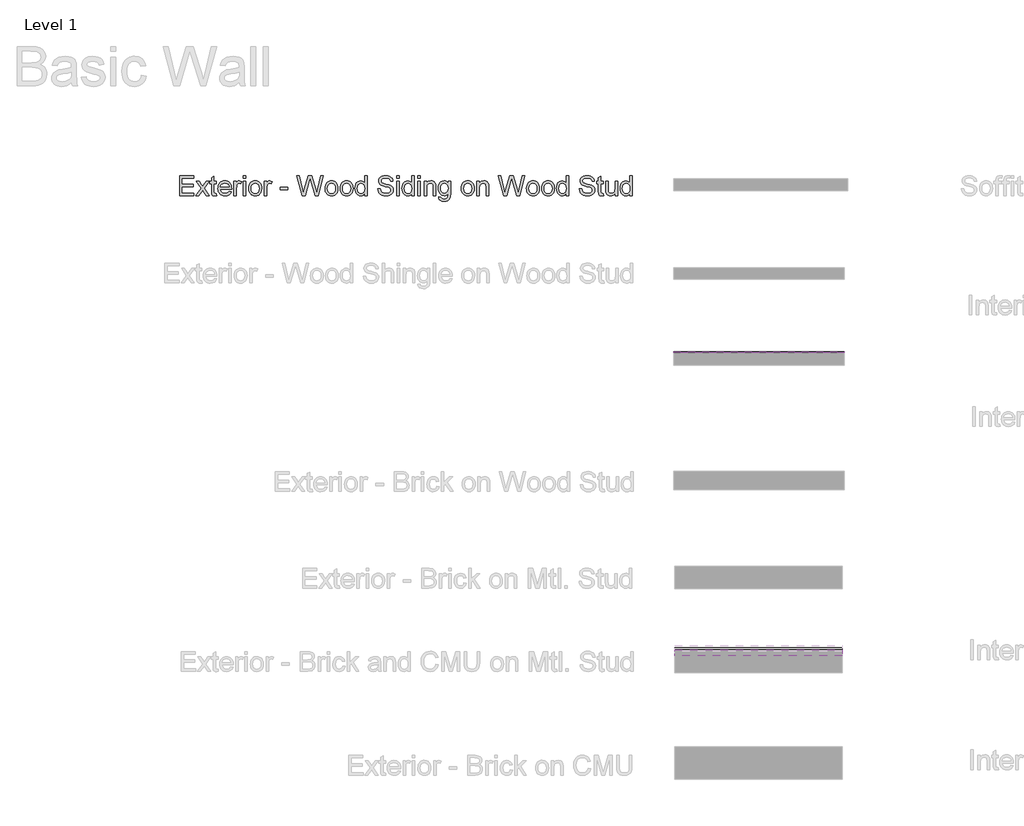
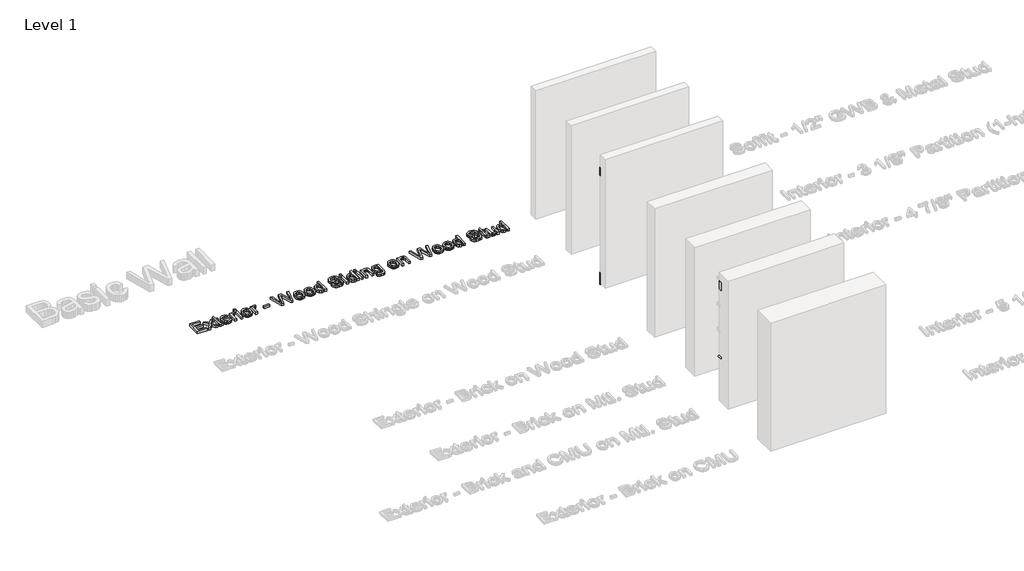
# One storey, part 31 of 42: 5 proxies.
"""IFC4 building model written with IfcOpenShell, lengths in millimetres."""

from ifc_helpers import new_model, si_unit, frame, origin, origin_with_axes, place, context, project, spatial, polyline, outline, extrude, faceted_brep, element, save

model = new_model("IFC4")

# Units and contexts
model_context = context("Model", 3, world=origin())
ifc_project = project(units=[si_unit("LENGTHUNIT", "METRE", prefix="MILLI")], contexts=[model_context])

# Site, building, storey
site = spatial("IfcSite", under=ifc_project)
building = spatial("IfcBuilding", under=site)
storey = spatial("IfcBuildingStorey", under=building, Name="Level 1", Elevation=0.0)

# Proxies
placement = place(None, origin())
element("IfcBuildingElementProxy", 1, Name="Wall Sweeps", at=placement, inside=storey, context=model_context, shape_type="Brep", body=[
    faceted_brep([(684.9886716, 10187.9507244, 1085.85), (684.9886716, 10280.0257244, 1085.85), (684.9886716, 10314.9507244, 1041.4), (684.9886716, 10314.9507244, 1016.0), (684.9886716, 10280.0257244, 1016.0), (684.9886716, 10187.9507244, 1016.0), (3275.7886716, 10187.9507244, 1085.85), (3275.7886716, 10187.9507244, 1016.0), (3275.7886716, 10280.0257244, 1016.0), (3275.7886716, 10314.9507244, 1016.0), (3275.7886716, 10314.9507244, 1041.4), (3275.7886716, 10280.0257244, 1085.85)], [[[0, 1, 2, 3, 4, 5]], [[6, 7, 8, 9, 10, 11]], [[1, 0, 6, 11]], [[2, 1, 11, 10]], [[3, 2, 10, 9]], [[5, 4, 3, 9, 8, 7]], [[0, 5, 7, 6]]]),
])
element("IfcBuildingElementProxy", 2, Name="Wall Sweeps", at=placement, inside=storey, context=model_context, shape_type="Brep", body=[
    faceted_brep([(684.9886716, 10280.0257244, 2844.8), (684.9886716, 10280.0257244, 2641.6), (684.9886716, 10187.9507244, 2641.6), (684.9886716, 10187.9507244, 2844.8), (684.9886716, 10254.6257244, 2844.8), (3275.7886716, 10280.0257244, 2844.8), (3275.7886716, 10254.6257244, 2844.8), (3275.7886716, 10187.9507244, 2844.8), (3275.7886716, 10187.9507244, 2641.6), (3275.7886716, 10280.0257244, 2641.6)], [[[0, 1, 2, 3, 4]], [[5, 6, 7, 8, 9]], [[1, 0, 5, 9]], [[2, 1, 9, 8]], [[3, 2, 8, 7]], [[0, 4, 3, 7, 6, 5]]]),
])
element("IfcBuildingElementProxy", 3, Name="Wall Sweeps", at=placement, inside=storey, context=model_context, shape_type="Brep", body=[
    faceted_brep([(668.8686716, 14892.2628373, 254.0), (668.8686716, 14892.2628373, -31.75), (668.8686716, 14873.2128373, -31.75), (668.8686716, 14873.2128373, 0.0), (668.8686716, 14873.2128373, 254.0), (3310.4686716, 14892.2628373, 254.0), (3310.4686716, 14873.2128373, 254.0), (3310.4686716, 14873.2128373, 0.0), (3310.4686716, 14873.2128373, -31.75), (3310.4686716, 14892.2628373, -31.75)], [[[0, 1, 2, 3, 4]], [[5, 6, 7, 8, 9]], [[1, 0, 5, 9]], [[2, 1, 9, 8]], [[4, 3, 2, 8, 7, 6]], [[0, 4, 6, 5]]]),
])
element("IfcBuildingElementProxy", 4, Name="Wall Sweeps", at=placement, inside=storey, context=model_context, shape_type="SweptSolid", body=[
    extrude(outline(polyline([(668.8686716, 14873.2128373), (668.8686716, 14892.2628373), (3310.4686716, 14892.2628373), (3310.4686716, 14873.2128373), (668.8686716, 14873.2128373)])), frame((0.0, 0.0, 2559.05), z_axis=(0.0, 0.0, 1.0), x_axis=(1.0, 0.0, 0.0)), (0.0, 0.0, 1.0), 184.15),
])
element("IfcBuildingElementProxy", 5, Name="8\" Arial", ObjectType="8\" Arial", at=placement, inside=storey, context=model_context, shape_type="SweptSolid", body=[
    extrude(outline(polyline([(-6977.0635915, 17307.3366547), (-6977.0635915, 17611.9037487), (-6758.1559926, 17611.9037487), (-6758.1559926, 17573.832862), (-6938.9927047, 17573.832862), (-6938.9927047, 17483.4145059), (-6767.6737143, 17483.4145059), (-6767.6737143, 17445.3436192), (-6938.9927047, 17445.3436192), (-6938.9927047, 17345.4075414), (-6753.3971318, 17345.4075414), (-6753.3971318, 17307.3366547), (-6977.0635915, 17307.3366547)])), origin_with_axes(), (0.0, 0.0, 1.0), 50.8),
    extrude(outline(polyline([(-6724.8439667, 17307.3366547), (-6643.4971892, 17419.7647421), (-6720.0851059, 17531.0031144), (-6674.2810702, 17531.0031144), (-6637.3255415, 17477.4659299), (-6620.0746709, 17452.1844816), (-6605.1288736, 17472.8557834), (-6563.042698, 17531.0031144), (-6517.2386624, 17531.0031144), (-6597.6931535, 17419.7647421), (-6520.2129504, 17307.3366547), (-6566.016986, 17307.3366547), (-6612.6389509, 17374.9273501), (-6621.1900289, 17387.2706454), (-6679.0399311, 17307.3366547), (-6724.8439667, 17307.3366547)])), origin_with_axes(), (0.0, 0.0, 1.0), 50.8),
    extrude(outline(polyline([(-6406.0002901, 17339.0871794), (-6401.2414293, 17306.2212967), (-6429.7202371, 17302.5777938), (-6447.9935192, 17304.1578843), (-6461.6194762, 17308.8981559), (-6471.2487337, 17316.2037509), (-6477.5319172, 17325.4798116), (-6480.989527, 17341.4108419), (-6482.1420636, 17368.6813453), (-6482.1420636, 17492.9322276), (-6510.6952287, 17492.9322276), (-6510.6952287, 17531.0031144), (-6482.1420636, 17531.0031144), (-6482.1420636, 17585.3582281), (-6444.0711769, 17607.7397455), (-6444.0711769, 17531.0031144), (-6406.0002901, 17531.0031144), (-6406.0002901, 17492.9322276), (-6444.0711769, 17492.9322276), (-6444.0711769, 17369.7967033), (-6442.0635325, 17350.1664023), (-6435.5572774, 17343.214004), (-6422.5819459, 17340.6486806), (-6406.0002901, 17339.0871794)])), origin_with_axes(), (0.0, 0.0, 1.0), 50.8),
    extrude(outline(polyline([(-6211.3331387, 17373.9607065), (-6174.0058239, 17369.2018457), (-6187.4551826, 17341.0762345), (-6208.9165297, 17320.051736), (-6237.9065433, 17306.9462794), (-6273.9419017, 17302.5777938), (-6297.5642549, 17304.4622841), (-6318.61199, 17310.1157551), (-6337.085107, 17319.5382066), (-6352.983606, 17332.7296387), (-6365.7683972, 17349.3229128), (-6374.9003909, 17368.9508901), (-6380.3795872, 17391.6135707), (-6382.2059859, 17417.3109545), (-6380.3609979, 17443.8797118), (-6374.8260337, 17467.2975827), (-6365.6010935, 17487.5645672), (-6352.6861772, 17504.6806653), (-6336.8295042, 17518.2787384), (-6318.7792937, 17527.9916478), (-6298.5355458, 17533.8193934), (-6276.0982605, 17535.7619752), (-6254.3836342, 17533.8240407), (-6234.7463623, 17528.0102371), (-6217.1864446, 17518.3205643), (-6201.7038812, 17504.7550225), (-6189.0654807, 17487.676103), (-6180.0380518, 17467.4462971), (-6174.6215945, 17444.0656048), (-6172.8161087, 17417.5340261), (-6173.0391803, 17407.2727324), (-6344.1350991, 17407.2727324), (-6337.5451922, 17378.7753352), (-6322.2369035, 17357.8251939), (-6300.1435203, 17344.9428089), (-6273.1983297, 17340.6486806), (-6252.9359925, 17342.6377357), (-6235.8710149, 17348.6049011), (-6222.003397, 17358.9219627), (-6211.3331387, 17373.9607065)]), holes=[polyline([(-6344.1350991, 17445.3436192), (-6210.8869955, 17445.3436192), (-6216.0362316, 17465.457242), (-6226.1302216, 17479.8453603), (-6248.325846, 17493.2296564), (-6276.2469749, 17497.6910885), (-6301.9095038, 17494.1312375), (-6323.1291899, 17483.4516845), (-6337.8797996, 17466.8049662), (-6344.1350991, 17445.3436192)])]), origin_with_axes(), (0.0, 0.0, 1.0), 50.8),
    extrude(outline(polyline([(-6134.745222, 17307.3366547), (-6134.745222, 17531.0031144), (-6101.433196, 17531.0031144), (-6101.433196, 17497.9141601), (-6089.1270793, 17517.0983178), (-6077.7876062, 17528.4006124), (-6066.4109545, 17533.9216345), (-6053.993302, 17535.7619752), (-6035.0322158, 17532.8248658), (-6015.7737008, 17524.0135375), (-6028.4887822, 17489.8835824), (-6041.8730783, 17495.7392119), (-6055.2573744, 17497.6910885), (-6066.6247315, 17495.8135691), (-6076.783784, 17490.1810112), (-6084.99096, 17481.2209685), (-6090.5026875, 17469.360995), (-6095.1314233, 17448.0948356), (-6096.6743352, 17424.895389), (-6096.6743352, 17307.3366547), (-6134.745222, 17307.3366547)])), origin_with_axes(), (0.0, 0.0, 1.0), 50.8),
    extrude(outline(polyline([(-5991.9793966, 17573.832862), (-5991.9793966, 17611.9037487), (-5953.9085099, 17611.9037487), (-5953.9085099, 17573.832862), (-5991.9793966, 17573.832862)])), origin_with_axes(), (0.0, 0.0, 1.0), 50.8),
    extrude(outline(polyline([(-5991.9793966, 17307.3366547), (-5991.9793966, 17531.0031144), (-5953.9085099, 17531.0031144), (-5953.9085099, 17307.3366547), (-5991.9793966, 17307.3366547)])), origin_with_axes(), (0.0, 0.0, 1.0), 50.8),
    extrude(outline(polyline([(-5906.3199014, 17419.1698845), (-5904.2611364, 17448.1366615), (-5898.0848414, 17473.0974443), (-5887.7910165, 17494.052233), (-5873.3796615, 17511.0010274), (-5858.8707127, 17521.8339421), (-5842.8560306, 17529.5717383), (-5825.3356152, 17534.214416), (-5806.3094665, 17535.7619752), (-5785.3058809, 17533.8774849), (-5766.3145871, 17528.224014), (-5749.3355851, 17518.8015625), (-5734.3688748, 17505.6101303), (-5722.1533809, 17489.0958608), (-5713.4280281, 17469.7048971), (-5708.1928165, 17447.4372391), (-5706.4477459, 17422.292887), (-5709.5335698, 17383.8316249), (-5718.7910412, 17354.5534771), (-5733.9506155, 17332.6273976), (-5754.7427478, 17316.2223402), (-5779.4386331, 17305.9889304), (-5806.3094665, 17302.5777938), (-5827.6197755, 17304.4553131), (-5846.7876676, 17310.0878711), (-5863.8131429, 17319.4754677), (-5878.6962014, 17332.6181029), (-5890.7815701, 17349.2927052), (-5899.4139764, 17369.2762029), (-5904.5934202, 17392.568596), (-5906.3199014, 17419.1698845)]), holes=[polyline([(-5868.2490147, 17419.2442417), (-5863.8433505, 17384.7889739), (-5850.6263581, 17360.241803), (-5830.7358069, 17345.5469612), (-5806.3094665, 17340.6486806), (-5781.9946618, 17345.5748451), (-5762.1412893, 17360.3533388), (-5748.9242968, 17385.2258224), (-5744.5186327, 17420.4339569), (-5748.9521808, 17453.8854026), (-5762.2528251, 17478.0979661), (-5782.1340816, 17492.7928079), (-5806.3094665, 17497.6910885), (-5830.7358069, 17492.8113972), (-5850.6263581, 17478.1723233), (-5863.8433505, 17453.6809203), (-5868.2490147, 17419.2442417)])]), origin_with_axes(), (0.0, 0.0, 1.0), 50.8),
    extrude(outline(polyline([(-5663.6179983, 17307.3366547), (-5663.6179983, 17531.0031144), (-5630.3059724, 17531.0031144), (-5630.3059724, 17497.9141601), (-5617.9998557, 17517.0983178), (-5606.6603826, 17528.4006124), (-5595.2837309, 17533.9216345), (-5582.8660784, 17535.7619752), (-5563.9049922, 17532.8248658), (-5544.6464772, 17524.0135375), (-5557.3615585, 17489.8835824), (-5570.7458547, 17495.7392119), (-5584.1301508, 17497.6910885), (-5595.4975078, 17495.8135691), (-5605.6565604, 17490.1810112), (-5613.8637364, 17481.2209685), (-5619.3754639, 17469.360995), (-5624.0041997, 17448.0948356), (-5625.5471116, 17424.895389), (-5625.5471116, 17307.3366547), (-5663.6179983, 17307.3366547)])), origin_with_axes(), (0.0, 0.0, 1.0), 50.8),
    extrude(outline(polyline([(-5420.9160952, 17397.7550107), (-5420.9160952, 17435.8258975), (-5301.9445741, 17435.8258975), (-5301.9445741, 17397.7550107), (-5420.9160952, 17397.7550107)])), origin_with_axes(), (0.0, 0.0, 1.0), 50.8),
    extrude(outline(polyline([(-5080.8806164, 17307.3366547), (-5163.9376096, 17611.9037487), (-5124.6770077, 17611.9037487), (-5076.4935416, 17411.7341645), (-5061.6221015, 17349.9433307), (-5045.7096605, 17404.5958732), (-4985.3316135, 17611.9037487), (-4928.7457838, 17611.9037487), (-4884.8750354, 17461.6278461), (-4866.0812529, 17405.8599456), (-4852.2322243, 17349.9433307), (-4837.8069273, 17409.9495916), (-4789.1773181, 17611.9037487), (-4749.9167161, 17611.9037487), (-4833.0480665, 17307.3366547), (-4873.7214553, 17307.3366547), (-4946.7402264, 17542.3054089), (-4956.9271629, 17575.0969344), (-4968.3781718, 17535.6132608), (-5034.9278664, 17307.3366547), (-5080.8806164, 17307.3366547)])), origin_with_axes(), (0.0, 0.0, 1.0), 50.8),
    extrude(outline(polyline([(-4726.1224119, 17419.1698845), (-4724.0636469, 17448.1366615), (-4717.8873519, 17473.0974443), (-4707.5935269, 17494.052233), (-4693.182172, 17511.0010274), (-4678.6732232, 17521.8339421), (-4662.6585411, 17529.5717383), (-4645.1381257, 17534.214416), (-4626.111977, 17535.7619752), (-4605.1083914, 17533.8774849), (-4586.1170976, 17528.224014), (-4569.1380956, 17518.8015625), (-4554.1713853, 17505.6101303), (-4541.9558914, 17489.0958608), (-4533.2305386, 17469.7048971), (-4527.995327, 17447.4372391), (-4526.2502564, 17422.292887), (-4529.3360802, 17383.8316249), (-4538.5935517, 17354.5534771), (-4553.753126, 17332.6273976), (-4574.5452583, 17316.2223402), (-4599.2411436, 17305.9889304), (-4626.111977, 17302.5777938), (-4647.4222859, 17304.4553131), (-4666.5901781, 17310.0878711), (-4683.6156534, 17319.4754677), (-4698.4987118, 17332.6181029), (-4710.5840806, 17349.2927052), (-4719.2164869, 17369.2762029), (-4724.3959306, 17392.568596), (-4726.1224119, 17419.1698845)]), holes=[polyline([(-4688.0515251, 17419.2442417), (-4683.645861, 17384.7889739), (-4670.4288686, 17360.241803), (-4650.5383174, 17345.5469612), (-4626.111977, 17340.6486806), (-4601.7971723, 17345.5748451), (-4581.9437997, 17360.3533388), (-4568.7268073, 17385.2258224), (-4564.3211432, 17420.4339569), (-4568.7546913, 17453.8854026), (-4582.0553355, 17478.0979661), (-4601.9365921, 17492.7928079), (-4626.111977, 17497.6910885), (-4650.5383174, 17492.8113972), (-4670.4288686, 17478.1723233), (-4683.645861, 17453.6809203), (-4688.0515251, 17419.2442417)])]), origin_with_axes(), (0.0, 0.0, 1.0), 50.8),
    extrude(outline(polyline([(-4492.9382305, 17419.1698845), (-4490.8794655, 17448.1366615), (-4484.7031705, 17473.0974443), (-4474.4093456, 17494.052233), (-4459.9979906, 17511.0010274), (-4445.4890418, 17521.8339421), (-4429.4743597, 17529.5717383), (-4411.9539443, 17534.214416), (-4392.9277956, 17535.7619752), (-4371.92421, 17533.8774849), (-4352.9329162, 17528.224014), (-4335.9539142, 17518.8015625), (-4320.9872039, 17505.6101303), (-4308.77171, 17489.0958608), (-4300.0463572, 17469.7048971), (-4294.8111456, 17447.4372391), (-4293.066075, 17422.292887), (-4296.1518988, 17383.8316249), (-4305.4093703, 17354.5534771), (-4320.5689446, 17332.6273976), (-4341.3610769, 17316.2223402), (-4366.0569622, 17305.9889304), (-4392.9277956, 17302.5777938), (-4414.2381045, 17304.4553131), (-4433.4059967, 17310.0878711), (-4450.431472, 17319.4754677), (-4465.3145304, 17332.6181029), (-4477.3998992, 17349.2927052), (-4486.0323055, 17369.2762029), (-4491.2117492, 17392.568596), (-4492.9382305, 17419.1698845)]), holes=[polyline([(-4454.8673437, 17419.2442417), (-4450.4616796, 17384.7889739), (-4437.2446872, 17360.241803), (-4417.354136, 17345.5469612), (-4392.9277956, 17340.6486806), (-4368.6129909, 17345.5748451), (-4348.7596183, 17360.3533388), (-4335.5426259, 17385.2258224), (-4331.1369618, 17420.4339569), (-4335.5705099, 17453.8854026), (-4348.8711541, 17478.0979661), (-4368.7524107, 17492.7928079), (-4392.9277956, 17497.6910885), (-4417.354136, 17492.8113972), (-4437.2446872, 17478.1723233), (-4450.4616796, 17453.6809203), (-4454.8673437, 17419.2442417)])]), origin_with_axes(), (0.0, 0.0, 1.0), 50.8),
    extrude(outline(polyline([(-4112.2293629, 17307.3366547), (-4112.2293629, 17343.2511826), (-4123.6199566, 17325.456575), (-4137.4178647, 17312.746141), (-4153.6230871, 17305.1198806), (-4172.2356239, 17302.5777938), (-4196.8478573, 17306.2584753), (-4219.3780891, 17317.3005196), (-4238.4507111, 17334.9324708), (-4252.690115, 17358.382873), (-4261.5572112, 17386.7036718), (-4264.5129099, 17418.9468129), (-4261.7895775, 17450.7902841), (-4253.61958, 17479.5479315), (-4240.0122123, 17503.5838966), (-4220.9767689, 17521.2623211), (-4197.9539207, 17532.1370617), (-4172.3843383, 17535.7619752), (-4153.7578595, 17533.1687679), (-4137.2877396, 17525.3891457), (-4123.3271751, 17513.4641097), (-4112.2293629, 17498.4346605), (-4112.2293629, 17611.9037487), (-4074.1584762, 17611.9037487), (-4074.1584762, 17307.3366547), (-4112.2293629, 17307.3366547)]), holes=[polyline([(-4226.4420232, 17419.0955273), (-4222.1478949, 17384.6588488), (-4209.2655098, 17360.1674458), (-4190.5460846, 17345.5283719), (-4168.7408354, 17340.6486806), (-4146.944881, 17345.3053003), (-4128.6994829, 17359.2751594), (-4116.3468929, 17382.818508), (-4112.2293629, 17416.1955965), (-4116.4212501, 17452.6863927), (-4128.9969117, 17477.9864303), (-4147.7070423, 17492.7649239), (-4170.3023367, 17497.6910885), (-4192.3306574, 17492.9601116), (-4210.3808678, 17478.7671809), (-4222.4267344, 17454.3873137), (-4226.4420232, 17419.0955273)])]), origin_with_axes(), (0.0, 0.0, 1.0), 50.8),
    extrude(outline(polyline([(-3907.5983466, 17412.0315933), (-3869.5274598, 17412.0315933), (-3865.1589743, 17390.9048536), (-3857.2585217, 17373.9235279), (-3844.9338157, 17360.4462853), (-3827.2925698, 17349.8317949), (-3805.7289816, 17342.9444592), (-3781.6372486, 17340.6486806), (-3760.4268571, 17342.3867802), (-3741.8561462, 17347.6010789), (-3726.8081077, 17355.8547281), (-3716.1657334, 17366.7108794), (-3709.8360767, 17379.1750052), (-3707.7261911, 17392.2525779), (-3709.3062816, 17404.9955431), (-3714.0465532, 17416.0097035), (-3723.6758107, 17425.4065947), (-3739.922859, 17433.2977527), (-3795.3561521, 17447.8345854), (-3831.7447072, 17457.4545482), (-3855.0278057, 17466.6097786), (-3873.9795972, 17479.4178064), (-3887.4103666, 17494.939872), (-3895.4130603, 17512.8413681), (-3898.0806249, 17532.7876872), (-3894.7810241, 17555.0855528), (-3884.8822218, 17575.877685), (-3868.6444681, 17593.5003416), (-3846.3280132, 17606.2897801), (-3819.5408317, 17614.0694022), (-3789.8908979, 17616.6626096), (-3757.7685872, 17613.9485718), (-3729.6615653, 17605.8064583), (-3706.5736545, 17592.4035729), (-3689.5086769, 17573.9072192), (-3678.7082935, 17551.4699339), (-3674.4141652, 17526.2442535), (-3712.485052, 17526.2442535), (-3719.4746288, 17548.9603784), (-3734.0486402, 17565.3561411), (-3756.8205329, 17575.2828274), (-3788.4037539, 17578.5917228), (-3820.7305469, 17575.320006), (-3842.907582, 17565.5048555), (-3855.7341991, 17551.0609693), (-3860.0097381, 17533.9030452), (-3856.9796822, 17519.273266), (-3847.8895144, 17507.506239), (-3826.4002834, 17496.9846951), (-3785.7268946, 17486.2400796), (-3743.7522548, 17476.0345538), (-3718.3592708, 17467.130279), (-3696.6562629, 17453.3184289), (-3681.5152779, 17436.2720407), (-3672.6202977, 17416.1770072), (-3669.6553043, 17393.2192215), (-3673.0664409, 17369.75023), (-3683.2998507, 17347.6754361), (-3699.9372743, 17328.6771713), (-3722.5604526, 17314.4377673), (-3749.7658935, 17305.5427872), (-3780.1501046, 17302.5777938), (-3817.4495354, 17305.7751535), (-3848.1497646, 17315.3672324), (-3872.603989, 17331.3912091), (-3891.1654052, 17353.8842623), (-3903.0811466, 17381.2848908), (-3907.5983466, 17412.0315933)])), origin_with_axes(), (0.0, 0.0, 1.0), 50.8),
    extrude(outline(polyline([(-3617.3078351, 17573.832862), (-3617.3078351, 17611.9037487), (-3579.2369483, 17611.9037487), (-3579.2369483, 17573.832862), (-3617.3078351, 17573.832862)])), origin_with_axes(), (0.0, 0.0, 1.0), 50.8),
    extrude(outline(polyline([(-3617.3078351, 17307.3366547), (-3617.3078351, 17531.0031144), (-3579.2369483, 17531.0031144), (-3579.2369483, 17307.3366547), (-3617.3078351, 17307.3366547)])), origin_with_axes(), (0.0, 0.0, 1.0), 50.8),
    extrude(outline(polyline([(-3384.1236537, 17307.3366547), (-3384.1236537, 17343.2511826), (-3395.5142473, 17325.456575), (-3409.3121554, 17312.746141), (-3425.5173778, 17305.1198806), (-3444.1299146, 17302.5777938), (-3468.7421481, 17306.2584753), (-3491.2723799, 17317.3005196), (-3510.3450018, 17334.9324708), (-3524.5844058, 17358.382873), (-3533.451502, 17386.7036718), (-3536.4072007, 17418.9468129), (-3533.6838682, 17450.7902841), (-3525.5138708, 17479.5479315), (-3511.9065031, 17503.5838966), (-3492.8710597, 17521.2623211), (-3469.8482114, 17532.1370617), (-3444.278629, 17535.7619752), (-3425.6521502, 17533.1687679), (-3409.1820303, 17525.3891457), (-3395.2214659, 17513.4641097), (-3384.1236537, 17498.4346605), (-3384.1236537, 17611.9037487), (-3346.0527669, 17611.9037487), (-3346.0527669, 17307.3366547), (-3384.1236537, 17307.3366547)]), holes=[polyline([(-3498.3363139, 17419.0955273), (-3494.0421856, 17384.6588488), (-3481.1598006, 17360.1674458), (-3462.4403753, 17345.5283719), (-3440.6351262, 17340.6486806), (-3418.8391717, 17345.3053003), (-3400.5937736, 17359.2751594), (-3388.2411836, 17382.818508), (-3384.1236537, 17416.1955965), (-3388.3155408, 17452.6863927), (-3400.8912024, 17477.9864303), (-3419.601333, 17492.7649239), (-3442.1966274, 17497.6910885), (-3464.2249481, 17492.9601116), (-3482.2751586, 17478.7671809), (-3494.3210251, 17454.3873137), (-3498.3363139, 17419.0955273)])]), origin_with_axes(), (0.0, 0.0, 1.0), 50.8),
    extrude(outline(polyline([(-3288.9464368, 17573.832862), (-3288.9464368, 17611.9037487), (-3250.87555, 17611.9037487), (-3250.87555, 17573.832862), (-3288.9464368, 17573.832862)])), origin_with_axes(), (0.0, 0.0, 1.0), 50.8),
    extrude(outline(polyline([(-3288.9464368, 17307.3366547), (-3288.9464368, 17531.0031144), (-3250.87555, 17531.0031144), (-3250.87555, 17307.3366547), (-3288.9464368, 17307.3366547)])), origin_with_axes(), (0.0, 0.0, 1.0), 50.8),
    extrude(outline(polyline([(-3193.7692199, 17307.3366547), (-3193.7692199, 17531.0031144), (-3155.6983331, 17531.0031144), (-3155.6983331, 17499.7730901), (-3142.472046, 17515.5182273), (-3126.587489, 17526.7647539), (-3108.0446621, 17533.5126699), (-3086.8435653, 17535.7619752), (-3068.0776667, 17533.9495185), (-3050.8918587, 17528.5121482), (-3036.5595083, 17520.1283738), (-3026.3539825, 17509.4767048), (-3014.9401522, 17481.4812187), (-3012.9325078, 17444.6744044), (-3012.9325078, 17307.3366547), (-3051.0033945, 17307.3366547), (-3051.0033945, 17439.5437575), (-3055.3904694, 17473.2275694), (-3061.4598759, 17483.2564969), (-3070.8939457, 17491.036119), (-3082.9862855, 17496.0273461), (-3097.0305018, 17497.6910885), (-3119.3283673, 17493.9546391), (-3138.3359267, 17482.7452911), (-3145.9319795, 17473.5947081), (-3151.3577315, 17461.0887564), (-3155.6983331, 17426.010747), (-3155.6983331, 17307.3366547), (-3193.7692199, 17307.3366547)])), origin_with_axes(), (0.0, 0.0, 1.0), 50.8),
    extrude(outline(polyline([(-2970.1027602, 17288.3012113), (-2932.0318734, 17283.5423505), (-2927.8306916, 17271.6451983), (-2919.6885781, 17263.4659063), (-2903.6831906, 17257.1083656), (-2882.7330493, 17254.9891854), (-2860.3887105, 17257.3872051), (-2843.7698762, 17264.5812643), (-2832.2445101, 17276.1066304), (-2825.180576, 17291.4985709), (-2822.578074, 17335.8898197), (-2835.246682, 17323.39781), (-2849.3838448, 17314.4749459), (-2864.9895623, 17309.1212275), (-2882.0638345, 17307.3366547), (-2902.937295, 17309.414009), (-2921.3151419, 17315.6460719), (-2937.1973752, 17326.0328433), (-2950.583995, 17340.5743234), (-2961.2054564, 17358.0203816), (-2968.7922145, 17377.1208875), (-2973.3442694, 17397.8758412), (-2974.861621, 17420.2852425), (-2972.1382885, 17451.0226504), (-2963.9682911, 17479.2876813), (-2950.6397629, 17503.2399946), (-2932.440838, 17521.0392495), (-2909.994258, 17532.0812938), (-2883.9227645, 17535.7619752), (-2866.1188623, 17533.6799736), (-2849.9601131, 17527.4339687), (-2835.446517, 17517.0239606), (-2822.578074, 17502.4499493), (-2822.578074, 17531.0031144), (-2784.5071872, 17531.0031144), (-2784.5071872, 17337.8974642), (-2787.1096892, 17293.3110277), (-2794.9171953, 17263.9492281), (-2808.366554, 17244.4769361), (-2827.8946138, 17229.5590227), (-2853.0738209, 17220.0784797), (-2883.4766213, 17216.9182986), (-2918.8985328, 17221.370436), (-2946.7917777, 17234.7268482), (-2957.297056, 17244.753452), (-2964.6839792, 17257.0247138), (-2968.9525472, 17271.5406335), (-2970.1027602, 17288.3012113)]), holes=[polyline([(-2936.7907342, 17422.8877446), (-2932.7289722, 17387.9677442), (-2920.5436859, 17363.959663), (-2902.2239306, 17350.0455718), (-2879.7587613, 17345.4075414), (-2857.4608957, 17350.0176879), (-2839.0481939, 17363.8481272), (-2826.695604, 17387.5494849), (-2822.578074, 17421.7723866), (-2826.8164344, 17454.777689), (-2839.5315157, 17478.5441093), (-2858.2137624, 17492.9043437), (-2880.3536189, 17497.6910885), (-2902.0938055, 17492.9787009), (-2920.3206143, 17478.8415381), (-2932.6732043, 17455.4283145), (-2936.7907342, 17422.8877446)])]), origin_with_axes(), (0.0, 0.0, 1.0), 50.8),
    extrude(outline(polyline([(-2617.9470576, 17419.1698845), (-2615.8882926, 17448.1366615), (-2609.7119977, 17473.0974443), (-2599.4181727, 17494.052233), (-2585.0068177, 17511.0010274), (-2570.4978689, 17521.8339421), (-2554.4831868, 17529.5717383), (-2536.9627714, 17534.214416), (-2517.9366227, 17535.7619752), (-2496.9330372, 17533.8774849), (-2477.9417434, 17528.224014), (-2460.9627413, 17518.8015625), (-2445.996031, 17505.6101303), (-2433.7805371, 17489.0958608), (-2425.0551844, 17469.7048971), (-2419.8199727, 17447.4372391), (-2418.0749022, 17422.292887), (-2421.160726, 17383.8316249), (-2430.4181975, 17354.5534771), (-2445.5777718, 17332.6273976), (-2466.369904, 17316.2223402), (-2491.0657893, 17305.9889304), (-2517.9366227, 17302.5777938), (-2539.2469317, 17304.4553131), (-2558.4148238, 17310.0878711), (-2575.4402991, 17319.4754677), (-2590.3233576, 17332.6181029), (-2602.4087264, 17349.2927052), (-2611.0411326, 17369.2762029), (-2616.2205764, 17392.568596), (-2617.9470576, 17419.1698845)]), holes=[polyline([(-2579.8761709, 17419.2442417), (-2575.4705067, 17384.7889739), (-2562.2535143, 17360.241803), (-2542.3629631, 17345.5469612), (-2517.9366227, 17340.6486806), (-2493.6218181, 17345.5748451), (-2473.7684455, 17360.3533388), (-2460.5514531, 17385.2258224), (-2456.1457889, 17420.4339569), (-2460.579337, 17453.8854026), (-2473.8799813, 17478.0979661), (-2493.7612378, 17492.7928079), (-2517.9366227, 17497.6910885), (-2542.3629631, 17492.8113972), (-2562.2535143, 17478.1723233), (-2575.4705067, 17453.6809203), (-2579.8761709, 17419.2442417)])]), origin_with_axes(), (0.0, 0.0, 1.0), 50.8),
    extrude(outline(polyline([(-2375.2451546, 17307.3366547), (-2375.2451546, 17531.0031144), (-2337.1742678, 17531.0031144), (-2337.1742678, 17499.7730901), (-2323.9479807, 17515.5182273), (-2308.0634237, 17526.7647539), (-2289.5205968, 17533.5126699), (-2268.3195, 17535.7619752), (-2249.5536014, 17533.9495185), (-2232.3677934, 17528.5121482), (-2218.035443, 17520.1283738), (-2207.8299172, 17509.4767048), (-2196.4160869, 17481.4812187), (-2194.4084425, 17444.6744044), (-2194.4084425, 17307.3366547), (-2232.4793292, 17307.3366547), (-2232.4793292, 17439.5437575), (-2236.8664041, 17473.2275694), (-2242.9358106, 17483.2564969), (-2252.3698804, 17491.036119), (-2264.4622202, 17496.0273461), (-2278.5064364, 17497.6910885), (-2300.804302, 17493.9546391), (-2319.8118614, 17482.7452911), (-2327.4079142, 17473.5947081), (-2332.8336662, 17461.0887564), (-2337.1742678, 17426.010747), (-2337.1742678, 17307.3366547), (-2375.2451546, 17307.3366547)])), origin_with_axes(), (0.0, 0.0, 1.0), 50.8),
    extrude(outline(polyline([(-1963.8267631, 17307.3366547), (-2046.8837563, 17611.9037487), (-2007.6231543, 17611.9037487), (-1959.4396882, 17411.7341645), (-1944.5682481, 17349.9433307), (-1928.6558072, 17404.5958732), (-1868.2777602, 17611.9037487), (-1811.6919305, 17611.9037487), (-1767.821182, 17461.6278461), (-1749.0273996, 17405.8599456), (-1735.1783709, 17349.9433307), (-1720.753074, 17409.9495916), (-1672.1234647, 17611.9037487), (-1632.8628628, 17611.9037487), (-1715.9942131, 17307.3366547), (-1756.6676019, 17307.3366547), (-1829.686373, 17542.3054089), (-1839.8733095, 17575.0969344), (-1851.3243184, 17535.6132608), (-1917.8740131, 17307.3366547), (-1963.8267631, 17307.3366547)])), origin_with_axes(), (0.0, 0.0, 1.0), 50.8),
    extrude(outline(polyline([(-1609.0685585, 17419.1698845), (-1607.0097935, 17448.1366615), (-1600.8334986, 17473.0974443), (-1590.5396736, 17494.052233), (-1576.1283186, 17511.0010274), (-1561.6193698, 17521.8339421), (-1545.6046877, 17529.5717383), (-1528.0842723, 17534.214416), (-1509.0581236, 17535.7619752), (-1488.0545381, 17533.8774849), (-1469.0632443, 17528.224014), (-1452.0842422, 17518.8015625), (-1437.1175319, 17505.6101303), (-1424.902038, 17489.0958608), (-1416.1766853, 17469.7048971), (-1410.9414736, 17447.4372391), (-1409.1964031, 17422.292887), (-1412.2822269, 17383.8316249), (-1421.5396984, 17354.5534771), (-1436.6992727, 17332.6273976), (-1457.4914049, 17316.2223402), (-1482.1872902, 17305.9889304), (-1509.0581236, 17302.5777938), (-1530.3684326, 17304.4553131), (-1549.5363247, 17310.0878711), (-1566.5618, 17319.4754677), (-1581.4448585, 17332.6181029), (-1593.5302273, 17349.2927052), (-1602.1626335, 17369.2762029), (-1607.3420773, 17392.568596), (-1609.0685585, 17419.1698845)]), holes=[polyline([(-1570.9976718, 17419.2442417), (-1566.5920076, 17384.7889739), (-1553.3750152, 17360.241803), (-1533.484464, 17345.5469612), (-1509.0581236, 17340.6486806), (-1484.743319, 17345.5748451), (-1464.8899464, 17360.3533388), (-1451.672954, 17385.2258224), (-1447.2672898, 17420.4339569), (-1451.7008379, 17453.8854026), (-1465.0014822, 17478.0979661), (-1484.8827387, 17492.7928079), (-1509.0581236, 17497.6910885), (-1533.484464, 17492.8113972), (-1553.3750152, 17478.1723233), (-1566.5920076, 17453.6809203), (-1570.9976718, 17419.2442417)])]), origin_with_axes(), (0.0, 0.0, 1.0), 50.8),
    extrude(outline(polyline([(-1375.8843771, 17419.1698845), (-1373.8256122, 17448.1366615), (-1367.6493172, 17473.0974443), (-1357.3554922, 17494.052233), (-1342.9441372, 17511.0010274), (-1328.4351884, 17521.8339421), (-1312.4205063, 17529.5717383), (-1294.9000909, 17534.214416), (-1275.8739422, 17535.7619752), (-1254.8703567, 17533.8774849), (-1235.8790629, 17528.224014), (-1218.9000608, 17518.8015625), (-1203.9333505, 17505.6101303), (-1191.7178566, 17489.0958608), (-1182.9925039, 17469.7048971), (-1177.7572922, 17447.4372391), (-1176.0122217, 17422.292887), (-1179.0980455, 17383.8316249), (-1188.355517, 17354.5534771), (-1203.5150913, 17332.6273976), (-1224.3072235, 17316.2223402), (-1249.0031088, 17305.9889304), (-1275.8739422, 17302.5777938), (-1297.1842512, 17304.4553131), (-1316.3521433, 17310.0878711), (-1333.3776186, 17319.4754677), (-1348.2606771, 17332.6181029), (-1360.3460459, 17349.2927052), (-1368.9784521, 17369.2762029), (-1374.1578959, 17392.568596), (-1375.8843771, 17419.1698845)]), holes=[polyline([(-1337.8134904, 17419.2442417), (-1333.4078262, 17384.7889739), (-1320.1908338, 17360.241803), (-1300.3002826, 17345.5469612), (-1275.8739422, 17340.6486806), (-1251.5591376, 17345.5748451), (-1231.705765, 17360.3533388), (-1218.4887726, 17385.2258224), (-1214.0831084, 17420.4339569), (-1218.5166565, 17453.8854026), (-1231.8173008, 17478.0979661), (-1251.6985573, 17492.7928079), (-1275.8739422, 17497.6910885), (-1300.3002826, 17492.8113972), (-1320.1908338, 17478.1723233), (-1333.4078262, 17453.6809203), (-1337.8134904, 17419.2442417)])]), origin_with_axes(), (0.0, 0.0, 1.0), 50.8),
    extrude(outline(polyline([(-995.1755096, 17307.3366547), (-995.1755096, 17343.2511826), (-1006.5661032, 17325.456575), (-1020.3640113, 17312.746141), (-1036.5692337, 17305.1198806), (-1055.1817705, 17302.5777938), (-1079.794004, 17306.2584753), (-1102.3242358, 17317.3005196), (-1121.3968577, 17334.9324708), (-1135.6362617, 17358.382873), (-1144.5033579, 17386.7036718), (-1147.4590566, 17418.9468129), (-1144.7357241, 17450.7902841), (-1136.5657267, 17479.5479315), (-1122.958359, 17503.5838966), (-1103.9229156, 17521.2623211), (-1080.9000673, 17532.1370617), (-1055.3304849, 17535.7619752), (-1036.7040062, 17533.1687679), (-1020.2338862, 17525.3891457), (-1006.2733218, 17513.4641097), (-995.1755096, 17498.4346605), (-995.1755096, 17611.9037487), (-957.1046228, 17611.9037487), (-957.1046228, 17307.3366547), (-995.1755096, 17307.3366547)]), holes=[polyline([(-1109.3881698, 17419.0955273), (-1105.0940415, 17384.6588488), (-1092.2116565, 17360.1674458), (-1073.4922312, 17345.5283719), (-1051.6869821, 17340.6486806), (-1029.8910276, 17345.3053003), (-1011.6456295, 17359.2751594), (-999.2930395, 17382.818508), (-995.1755096, 17416.1955965), (-999.3673967, 17452.6863927), (-1011.9430583, 17477.9864303), (-1030.6531889, 17492.7649239), (-1053.2484833, 17497.6910885), (-1075.276804, 17492.9601116), (-1093.3270145, 17478.7671809), (-1105.372881, 17454.3873137), (-1109.3881698, 17419.0955273)])]), origin_with_axes(), (0.0, 0.0, 1.0), 50.8),
    extrude(outline(polyline([(-790.5444932, 17412.0315933), (-752.4736065, 17412.0315933), (-748.1051209, 17390.9048536), (-740.2046684, 17373.9235279), (-727.8799623, 17360.4462853), (-710.2387165, 17349.8317949), (-688.6751283, 17342.9444592), (-664.5833952, 17340.6486806), (-643.3730037, 17342.3867802), (-624.8022929, 17347.6010789), (-609.7542544, 17355.8547281), (-599.11188, 17366.7108794), (-592.7822233, 17379.1750052), (-590.6723378, 17392.2525779), (-592.2524283, 17404.9955431), (-596.9926998, 17416.0097035), (-606.6219573, 17425.4065947), (-622.8690057, 17433.2977527), (-678.3022988, 17447.8345854), (-714.6908539, 17457.4545482), (-737.9739523, 17466.6097786), (-756.9257439, 17479.4178064), (-770.3565132, 17494.939872), (-778.359207, 17512.8413681), (-781.0267715, 17532.7876872), (-777.7271708, 17555.0855528), (-767.8283684, 17575.877685), (-751.5906147, 17593.5003416), (-729.2741599, 17606.2897801), (-702.4869783, 17614.0694022), (-672.8370445, 17616.6626096), (-640.7147338, 17613.9485718), (-612.607712, 17605.8064583), (-589.5198011, 17592.4035729), (-572.4548236, 17573.9072192), (-561.6544402, 17551.4699339), (-557.3603118, 17526.2442535), (-595.4311986, 17526.2442535), (-602.4207755, 17548.9603784), (-616.9947868, 17565.3561411), (-639.7666795, 17575.2828274), (-671.3499005, 17578.5917228), (-703.6766935, 17575.320006), (-725.8537286, 17565.5048555), (-738.6803457, 17551.0609693), (-742.9558848, 17533.9030452), (-739.9258289, 17519.273266), (-730.8356611, 17507.506239), (-709.3464301, 17496.9846951), (-668.6730413, 17486.2400796), (-626.6984015, 17476.0345538), (-601.3054175, 17467.130279), (-579.6024095, 17453.3184289), (-564.4614245, 17436.2720407), (-555.5664444, 17416.1770072), (-552.601451, 17393.2192215), (-556.0125876, 17369.75023), (-566.2459973, 17347.6754361), (-582.883421, 17328.6771713), (-605.5065993, 17314.4377673), (-632.7120401, 17305.5427872), (-663.0962512, 17302.5777938), (-700.395682, 17305.7751535), (-731.0959113, 17315.3672324), (-755.5501357, 17331.3912091), (-774.1115519, 17353.8842623), (-786.0272933, 17381.2848908), (-790.5444932, 17412.0315933)])), origin_with_axes(), (0.0, 0.0, 1.0), 50.8),
    extrude(outline(polyline([(-419.3533473, 17339.0871794), (-414.5944865, 17306.2212967), (-443.0732944, 17302.5777938), (-461.3465764, 17304.1578843), (-474.9725335, 17308.8981559), (-484.601791, 17316.2037509), (-490.8849744, 17325.4798116), (-494.3425842, 17341.4108419), (-495.4951209, 17368.6813453), (-495.4951209, 17492.9322276), (-524.0482859, 17492.9322276), (-524.0482859, 17531.0031144), (-495.4951209, 17531.0031144), (-495.4951209, 17585.3582281), (-457.4242341, 17607.7397455), (-457.4242341, 17531.0031144), (-419.3533473, 17531.0031144), (-419.3533473, 17492.9322276), (-457.4242341, 17492.9322276), (-457.4242341, 17369.7967033), (-455.4165897, 17350.1664023), (-448.9103346, 17343.214004), (-435.9350031, 17340.6486806), (-419.3533473, 17339.0871794)])), origin_with_axes(), (0.0, 0.0, 1.0), 50.8),
    extrude(outline(polyline([(-238.5166352, 17307.3366547), (-238.5166352, 17345.7793274), (-252.2913067, 17326.8786565), (-268.3338727, 17313.3781772), (-286.6443334, 17305.2778897), (-307.2226887, 17302.5777938), (-325.7655156, 17304.4739024), (-343.0256808, 17310.1622283), (-357.5067457, 17318.7133064), (-367.7122715, 17329.1976717), (-374.5810179, 17341.9313423), (-379.0517446, 17357.2303363), (-381.2824606, 17392.6243639), (-381.2824606, 17531.0031144), (-343.2115738, 17531.0031144), (-343.2115738, 17410.5444492), (-340.9065006, 17371.7299905), (-335.3575945, 17358.7825429), (-325.8491675, 17348.9395085), (-313.0132557, 17342.7213876), (-297.4818954, 17340.6486806), (-281.0582487, 17342.7678608), (-265.6941921, 17349.1254015), (-253.025584, 17359.1357396), (-244.6882829, 17372.2133123), (-240.0595471, 17390.124103), (-238.5166352, 17414.6340953), (-238.5166352, 17531.0031144), (-200.4457485, 17531.0031144), (-200.4457485, 17307.3366547), (-238.5166352, 17307.3366547)])), origin_with_axes(), (0.0, 0.0, 1.0), 50.8),
    extrude(outline(polyline([(-10.0913147, 17307.3366547), (-10.0913147, 17343.2511826), (-21.4819084, 17325.456575), (-35.2798164, 17312.746141), (-51.4850388, 17305.1198806), (-70.0975756, 17302.5777938), (-94.7098091, 17306.2584753), (-117.2400409, 17317.3005196), (-136.3126629, 17334.9324708), (-150.5520668, 17358.382873), (-159.419163, 17386.7036718), (-162.3748617, 17418.9468129), (-159.6515292, 17450.7902841), (-151.4815318, 17479.5479315), (-137.8741641, 17503.5838966), (-118.8387207, 17521.2623211), (-95.8158724, 17532.1370617), (-70.24629, 17535.7619752), (-51.6198113, 17533.1687679), (-35.1496913, 17525.3891457), (-21.1891269, 17513.4641097), (-10.0913147, 17498.4346605), (-10.0913147, 17611.9037487), (27.9795721, 17611.9037487), (27.9795721, 17307.3366547), (-10.0913147, 17307.3366547)]), holes=[polyline([(-124.303975, 17419.0955273), (-120.0098466, 17384.6588488), (-107.1274616, 17360.1674458), (-88.4080363, 17345.5283719), (-66.6027872, 17340.6486806), (-44.8068328, 17345.3053003), (-26.5614346, 17359.2751594), (-14.2088447, 17382.818508), (-10.0913147, 17416.1955965), (-14.2832019, 17452.6863927), (-26.8588634, 17477.9864303), (-45.5689941, 17492.7649239), (-68.1642884, 17497.6910885), (-90.1926091, 17492.9601116), (-108.2428196, 17478.7671809), (-120.2886861, 17454.3873137), (-124.303975, 17419.0955273)])]), origin_with_axes(), (0.0, 0.0, 1.0), 50.8),
])

save(model, "model.ifc")

# Revit data of these elements
# Element 1 (IfcBuildingElementProxy)
#   Phase Created = New Construction
#   Materials on its faces: "Concrete, Precast"
# Element 2 (IfcBuildingElementProxy)
#   Phase Created = New Construction
#   Materials on its faces: "Brick, Soldier Course"
# Element 3 (IfcBuildingElementProxy)
#   Phase Created = New Construction
#   Materials on its faces: "Wood Shake"
# Element 4 (IfcBuildingElementProxy)
#   Phase Created = New Construction
#   Materials on its faces: "Pine"
# Element 5 (IfcBuildingElementProxy, "8\" Arial")
#   Phase Created = New Construction
# Materials
#   "Concrete, Precast": class "Concrete", colour RGB 198 187 187, transparency 0, Description = "Precast concrete", Cost = 0
#   "Brick, Soldier Course": class "Masonry", colour RGB 170 98 104, transparency 0, Description = "Common brick soldier coursed", Cost = 0
#   "Wood Shake": class "Wood", colour RGB 151 131 103, transparency 0, Description = "Wood roofing shakes", Cost = 0
#   "Pine": class "Wood", colour RGB 223 192 134, transparency 0, Description = "Pinus Echinata", Cost = 0
